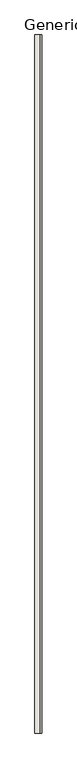
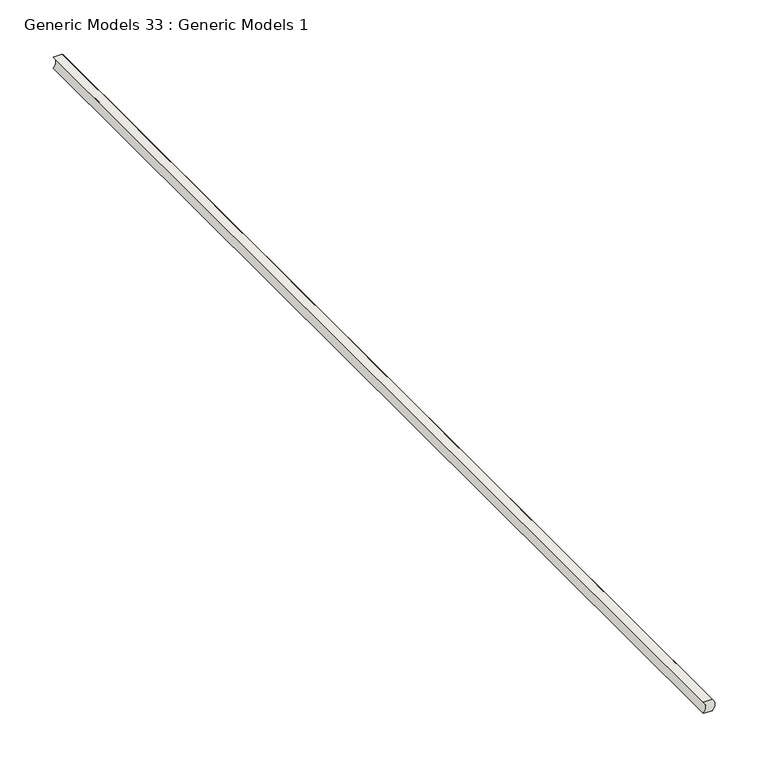
"""IFC4 building model written with IfcOpenShell, lengths in millimetres: wall geometry, Generic Models 33 : Generic Models 1."""

import ifcopenshell
import ifcopenshell.guid

model = None  # the IFC model being written
_history = None  # IfcOwnerHistory: only IFC2X3 demands one
_inside = {}  # id of a spatial element -> (the spatial element, [elements in it])
_under = {}  # id of a project, library or spatial element -> (it, [spatial elements below it])
_declared = {}  # id of a project -> (the project, [libraries it declares])
_typed = {}  # id of a type object -> (the type object, [elements of that type])
_made_of = {}  # id of a material, layer set ... -> (it, [elements and type objects made of it])


def new_model(schema):
    """Start an empty IFC model of exactly this schema.

    Asked for "IFC4X3", IfcOpenShell would pick the latest addendum, in which some entities
    have other attributes; the version numbers below select the first issue.
    IFC2X3 requires an IfcOwnerHistory on every rooted entity: one is made here for all.
    """
    global model, _history
    if schema == "IFC4X3":
        model = ifcopenshell.file(schema_version=(4, 3, 0, 0))
    else:
        model = ifcopenshell.file(schema=schema)
    _inside.clear()
    _under.clear()
    _declared.clear()
    _typed.clear()
    _made_of.clear()
    _history = None
    if model.schema == "IFC2X3":
        org = make("IfcOrganization", Name="unknown")
        user = make(
            "IfcPersonAndOrganization",
            ThePerson=make("IfcPerson", FamilyName="unknown"),
            TheOrganization=org,
        )
        app = make(
            "IfcApplication",
            ApplicationDeveloper=org,
            Version="unknown",
            ApplicationFullName="unknown",
            ApplicationIdentifier="unknown",
        )
        _history = make(
            "IfcOwnerHistory",
            OwningUser=user,
            OwningApplication=app,
            ChangeAction="ADDED",
            CreationDate=0,
        )
    return model


def make(cls, **values):
    """One entity of the class cls with the attributes given. An attribute that is None is left unset."""
    return model.create_entity(
        cls, **{name: value for name, value in values.items() if value is not None}
    )


def rooted(cls, **values):
    """An entity with a GlobalId (a new one), such as an element, a storey or a relation."""
    return make(cls, GlobalId=ifcopenshell.guid.new(), OwnerHistory=_history, **values)


def si_unit(unit_type, name, prefix=None):
    """IfcSIUnit, for example si_unit("LENGTHUNIT", "METRE", prefix="MILLI")."""
    return make("IfcSIUnit", UnitType=unit_type, Prefix=prefix, Name=name)


def assignment(units):
    """IfcUnitAssignment: the units of a project."""
    return None if units is None else make("IfcUnitAssignment", Units=units)


def point(xyz):
    """IfcCartesianPoint."""
    return None if xyz is None else make("IfcCartesianPoint", Coordinates=xyz)


def direction(xyz):
    """IfcDirection."""
    return None if xyz is None else make("IfcDirection", DirectionRatios=xyz)


def frame(location, z_axis=None, x_axis=None):
    """IfcAxis2Placement3D, a coordinate frame: its origin and axes. An axis left out is left unset."""
    return make(
        "IfcAxis2Placement3D",
        Location=point(location),
        Axis=direction(z_axis),
        RefDirection=direction(x_axis),
    )


def frame_2d(location, x_axis=None):
    """IfcAxis2Placement2D, a coordinate frame in the plane: its origin and x axis."""
    return make(
        "IfcAxis2Placement2D", Location=point(location), RefDirection=direction(x_axis)
    )


def origin():
    """The frame at (0, 0, 0) with its axes left unset."""
    return frame((0.0, 0.0, 0.0))


def place(relative_to, where):
    """IfcLocalPlacement: puts the frame where relative to a parent placement (None: the world)."""
    return make(
        "IfcLocalPlacement", PlacementRelTo=relative_to, RelativePlacement=where
    )


def context(
    kind, dimensions, precision=None, world=None, true_north=None, identifier=None
):
    """IfcGeometricRepresentationContext, for example the 3D "Model" context."""
    return make(
        "IfcGeometricRepresentationContext",
        ContextIdentifier=identifier,
        ContextType=kind,
        CoordinateSpaceDimension=dimensions,
        Precision=precision,
        WorldCoordinateSystem=world,
        TrueNorth=true_north,
    )


def project(units=None, contexts=None):
    """IfcProject with its units and contexts."""
    return rooted(
        "IfcProject",
        Name="project",
        RepresentationContexts=contexts,
        UnitsInContext=assignment(units),
    )


def spatial(cls, under=None, at=None, **own):
    """A site, building, storey or space (cls), placed at a placement, below another one or the project."""
    s = rooted(cls, ObjectPlacement=at, **own)
    if under is not None:
        _under.setdefault(under.id(), (under, []))[1].append(s)
    return s


def polyline(points):
    """IfcPolyline through the points."""
    return make("IfcPolyline", Points=[point(p) for p in points])


def circle_curve(where, radius):
    """IfcCircle in the frame where."""
    return make("IfcCircle", Position=where, Radius=radius)


def trimmed(basis, trim1, trim2, sense, master):
    """IfcTrimmedCurve: the piece of a basis curve between two trims."""
    return make(
        "IfcTrimmedCurve",
        BasisCurve=basis,
        Trim1=trim1,
        Trim2=trim2,
        SenseAgreement=sense,
        MasterRepresentation=master,
    )


def segment(curve, same_sense, transition):
    """IfcCompositeCurveSegment."""
    return make(
        "IfcCompositeCurveSegment",
        Transition=transition,
        SameSense=same_sense,
        ParentCurve=curve,
    )


def composite_curve(segments, self_intersect=None):
    """IfcCompositeCurve: segments joined end to end."""
    return make("IfcCompositeCurve", Segments=segments, SelfIntersect=self_intersect)


def outline(outer, holes=None, kind="AREA"):
    """IfcArbitraryClosedProfileDef: a profile drawn as a closed curve; with holes, ...WithVoids."""
    if holes is None:
        return make("IfcArbitraryClosedProfileDef", ProfileType=kind, OuterCurve=outer)
    return make(
        "IfcArbitraryProfileDefWithVoids",
        ProfileType=kind,
        OuterCurve=outer,
        InnerCurves=holes,
    )


def extrude(swept, where, along, depth):
    """IfcExtrudedAreaSolid: the profile swept, set in the frame where, extruded along a direction by depth."""
    return make(
        "IfcExtrudedAreaSolid",
        SweptArea=swept,
        Position=where,
        ExtrudedDirection=direction(along),
        Depth=depth,
    )


def shape(context_of_items, identifier, shape_type, items):
    """IfcShapeRepresentation: the items that make up one representation, for example the "Body"."""
    return make(
        "IfcShapeRepresentation",
        ContextOfItems=context_of_items,
        RepresentationIdentifier=identifier,
        RepresentationType=shape_type,
        Items=items,
    )


def source(mapping_origin, context_of_items, identifier, shape_type, items):
    """IfcRepresentationMap: a shape defined once, which mapped items show again and again."""
    return make(
        "IfcRepresentationMap",
        MappingOrigin=mapping_origin,
        MappedRepresentation=shape(context_of_items, identifier, shape_type, items),
    )


def transform(
    local_origin,
    x_axis=None,
    y_axis=None,
    z_axis=None,
    scale=None,
    scale2=None,
    scale3=None,
    uniform=True,
):
    """IfcCartesianTransformationOperator3D, or its non-uniform kind. x_axis, y_axis, z_axis: its Axis1, 2, 3."""
    if uniform:
        return make(
            "IfcCartesianTransformationOperator3D",
            Axis1=direction(x_axis),
            Axis2=direction(y_axis),
            LocalOrigin=point(local_origin),
            Scale=scale,
            Axis3=direction(z_axis),
        )
    return make(
        "IfcCartesianTransformationOperator3DnonUniform",
        Axis1=direction(x_axis),
        Axis2=direction(y_axis),
        LocalOrigin=point(local_origin),
        Scale=scale,
        Axis3=direction(z_axis),
        Scale2=scale2,
        Scale3=scale3,
    )


def mapped(mapping_source, mapping_target):
    """IfcMappedItem: shows the shape of a source again, moved by a transform."""
    return make(
        "IfcMappedItem", MappingSource=mapping_source, MappingTarget=mapping_target
    )


def made_of(thing, what):
    """Note that an element or type object is made of a material, layer set ...; save() writes the relation."""
    if what is not None:
        _made_of.setdefault(what.id(), (what, []))[1].append(thing)
    return thing


def element(
    cls,
    number,
    at=None,
    inside=None,
    cuts=None,
    type_object=None,
    material=None,
    context=None,
    identifier="Body",
    shape_type=None,
    held_by="IfcProductDefinitionShape",
    body=None,
    shapes=None,
    **own,
):
    """One element of the class cls, such as IfcWall. Its Tag is "e" and its number.

    at: its placement. inside: the storey or other place that contains it. cuts: it is an
    opening in that element (IfcRelVoidsElement). A single representation is given by context,
    identifier, shape_type and body (its items); several are given by shapes. held_by: the class
    of the entity that holds the representations. save() writes the other relations.
    """
    e = rooted(cls, Tag="e%d" % number, ObjectPlacement=at, **own)
    if body is not None:
        shapes = [shape(context, identifier, shape_type, body)]
    if shapes is not None:
        e.Representation = make(held_by, Representations=shapes)
    if inside is not None:
        _inside.setdefault(inside.id(), (inside, []))[1].append(e)
    if cuts is not None:
        rooted(
            "IfcRelVoidsElement", RelatingBuildingElement=cuts, RelatedOpeningElement=e
        )
    if type_object is not None:
        _typed.setdefault(type_object.id(), (type_object, []))[1].append(e)
    return made_of(e, material)


def aggregate(whole, parts):
    """IfcRelAggregates: a whole, such as a stair, and the parts it consists of."""
    return rooted("IfcRelAggregates", RelatingObject=whole, RelatedObjects=parts)


def save(model, path):
    """Write the relations noted so far, then the file.

    IfcRelAggregates (storeys below a building ...), IfcRelContainedInSpatialStructure (elements
    in a storey), IfcRelDefinesByType, IfcRelAssociatesMaterial and IfcRelDeclares: one each for
    every whole, place, type object, material and project.
    """
    for whole, parts in _under.values():
        aggregate(whole, parts)
    for where, things in _inside.values():
        rooted(
            "IfcRelContainedInSpatialStructure",
            RelatedElements=things,
            RelatingStructure=where,
        )
    for kind, things in _typed.values():
        rooted("IfcRelDefinesByType", RelatedObjects=things, RelatingType=kind)
    for what, things in _made_of.values():
        rooted("IfcRelAssociatesMaterial", RelatedObjects=things, RelatingMaterial=what)
    for by, libraries in _declared.values():
        rooted("IfcRelDeclares", RelatingContext=by, RelatedDefinitions=libraries)
    model.write(path)


def generic_models_33_generic_models_1_857ea60f(model_context):
    return source(origin(), model_context, "Body", "SweptSolid", [
        extrude(outline(composite_curve([segment(polyline([(2444.75, 141116.05), (2444.75, 141125.575)]), True, "CONTINUOUS"), segment(trimmed(circle_curve(frame_2d((2451.1, 141119.745519)), 8.620055), [point((2444.75, 141125.575))], [point((2457.45, 141125.575))], False, "CARTESIAN"), True, "CONTINUOUS"), segment(polyline([(2457.45, 141125.575), (2457.45, 141116.05)]), True, "CONTINUOUS"), segment(trimmed(circle_curve(frame_2d((2451.1, 141110.220519)), 8.620055), [point((2457.45, 141116.05))], [point((2444.75, 141116.05))], True, "CARTESIAN"), True, "CONTINUOUS")], self_intersect=False)), frame((0.0, 0.0, 0.0), z_axis=(0.0, 1.0, 0.0), x_axis=(0.0, 0.0, 1.0)), (0.0, 0.0, 1.0), 1219.2),
    ])


if __name__ == "__main__":
    model = new_model("IFC4")
    model_context = context("Model", 3, world=origin())
    ifc_project = project(units=[si_unit("LENGTHUNIT", "METRE", prefix="MILLI")], contexts=[model_context])
    site = spatial("IfcSite", under=ifc_project)
    building = spatial("IfcBuilding", under=site)
    placement = place(None, origin())
    generic_models_33_generic_models_1_shape = generic_models_33_generic_models_1_857ea60f(model_context)
    element("IfcWall", 1, ObjectType="Generic Models 33 : Generic Models 1", at=placement, inside=building, context=model_context, shape_type="MappedRepresentation", body=[
        mapped(generic_models_33_generic_models_1_shape, transform((0.0, 0.0, 0.0), x_axis=(1.0, 0.0, 0.0), y_axis=(0.0, 1.0, 0.0), z_axis=(0.0, 0.0, 1.0))),
    ])
    save(model, "model.ifc")

# Revit data of these elements
# Element 1 (IfcWall, "Generic Models 33 : Generic Models 1")
#   Materials on its faces: "ACOUSTICAL SEALANT OR FIRE SEALANT, IF RATED WALL"
# Materials
#   "ACOUSTICAL SEALANT OR FIRE SEALANT, IF RATED WALL": class "Unassigned", colour RGB 120 120 120, transparency 0, Cost = 0
